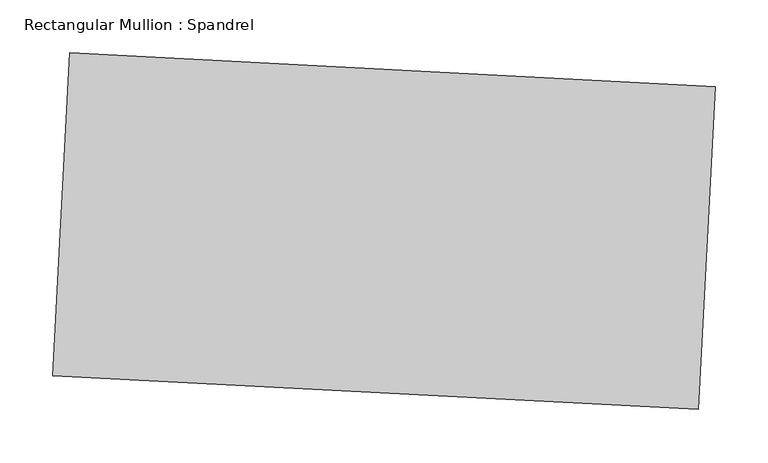
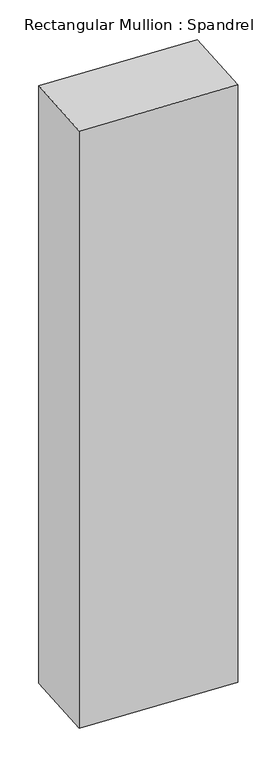
"""IFC4 building model written with IfcOpenShell, lengths in millimetres: member geometry, Rectangular Mullion : Spandrel."""

from ifc_helpers import new_model, si_unit, frame, origin, place, context, project, spatial, polyline, outline, extrude, source, transform, mapped, element, save


def rectangular_mullion_spandrel_52f45183(model_context):
    return source(origin(), model_context, "Body", "SweptSolid", [
        extrude(outline(polyline([(312.3582819, 136.2391416), (296.4062825, -168.1431406), (-312.3582819, -136.2391416), (-296.4062825, 168.1431406), (312.3582819, 136.2391416)])), frame((0.0, 0.0, -2501.3782228), z_axis=(0.0, 0.0, 1.0), x_axis=(1.0, 0.0, 0.0)), (0.0, 0.0, 1.0), 2501.3782228),
    ])


if __name__ == "__main__":
    model = new_model("IFC4")
    model_context = context("Model", 3, world=origin())
    ifc_project = project(units=[si_unit("LENGTHUNIT", "METRE", prefix="MILLI")], contexts=[model_context])
    site = spatial("IfcSite", under=ifc_project)
    building = spatial("IfcBuilding", under=site)
    placement = place(None, origin())
    rectangular_mullion_spandrel_shape = rectangular_mullion_spandrel_52f45183(model_context)
    element("IfcMember", 1, ObjectType="Rectangular Mullion : Spandrel", at=placement, inside=building, context=model_context, shape_type="MappedRepresentation", body=[
        mapped(rectangular_mullion_spandrel_shape, transform((0.0, 0.0, 0.0), x_axis=(1.0, 0.0, 0.0), y_axis=(0.0, 1.0, 0.0), z_axis=(0.0, 0.0, 1.0))),
    ])
    save(model, "model.ifc")

# Revit data of these elements
# Type "Rectangular Mullion : Spandrel"
#   built-in parameter 1007304 = 1 (stored number, unit not read)
#   built-in parameter 1007301 = 1 (stored number, unit not read)
#   built-in parameter 1007300 = 1 (stored number, unit not read)
# Element 1 (IfcMember, "Rectangular Mullion : Spandrel")
#   Materials on its faces: "Aluminum"
# Materials
#   "Aluminum": class "Metal", colour RGB 247 247 247, transparency 0, Description = "Aluminum 6061", Cost = 0
